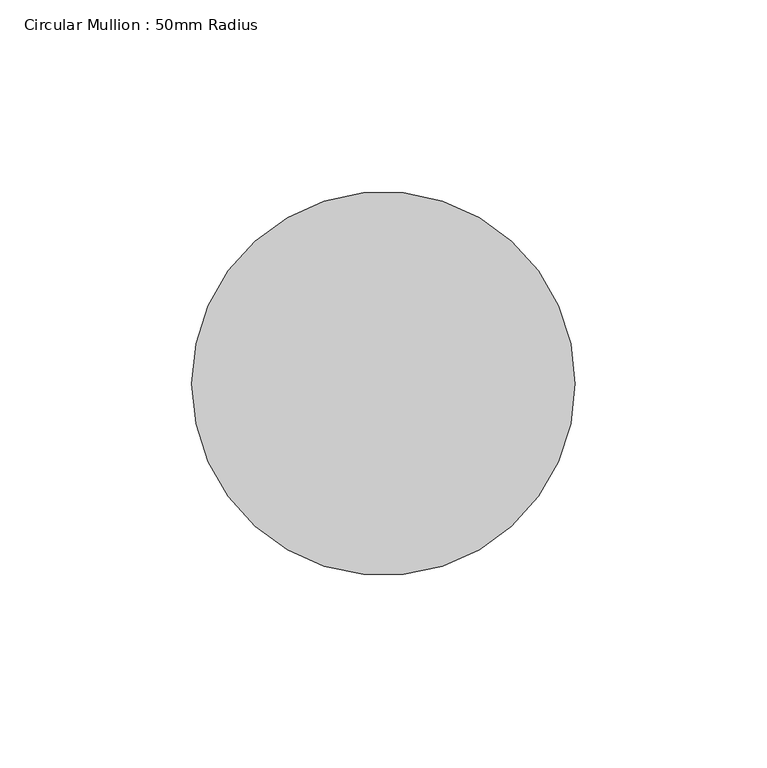
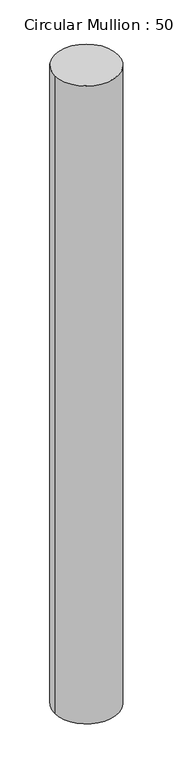
"""IFC4 building model written with IfcOpenShell, lengths in millimetres: member geometry, Circular Mullion : 50mm Radius."""

from ifc_helpers import new_model, si_unit, point, frame, origin, origin_2d, place, context, project, spatial, circle_curve, trimmed, segment, composite_curve, outline, extrude, source, transform, mapped, element, save


def circular_mullion_50mm_radius_614d2024(model_context):
    return source(origin(), model_context, "Body", "SweptSolid", [
        extrude(outline(composite_curve([segment(trimmed(circle_curve(origin_2d(), 50.0), [point((50.0, 0.0))], [point((-50.0, 0.0))], False, "CARTESIAN"), True, "CONTINUOUS"), segment(trimmed(circle_curve(origin_2d(), 50.0), [point((-50.0, 0.0))], [point((50.0, 0.0))], False, "CARTESIAN"), True, "CONTINUOUS")], self_intersect=False)), frame((0.0, 0.0, -1066.8394023), z_axis=(0.0, 0.0, 1.0), x_axis=(1.0, 0.0, 0.0)), (0.0, 0.0, 1.0), 1066.8394023),
    ])


if __name__ == "__main__":
    model = new_model("IFC4")
    model_context = context("Model", 3, world=origin())
    ifc_project = project(units=[si_unit("LENGTHUNIT", "METRE", prefix="MILLI")], contexts=[model_context])
    site = spatial("IfcSite", under=ifc_project)
    building = spatial("IfcBuilding", under=site)
    placement = place(None, origin())
    circular_mullion_50mm_radius_shape = circular_mullion_50mm_radius_614d2024(model_context)
    element("IfcMember", 1, ObjectType="Circular Mullion : 50mm Radius", at=placement, inside=building, context=model_context, shape_type="MappedRepresentation", body=[
        mapped(circular_mullion_50mm_radius_shape, transform((0.0, 0.0, 0.0), x_axis=(1.0, 0.0, 0.0), y_axis=(0.0, 1.0, 0.0), z_axis=(0.0, 0.0, 1.0))),
    ])
    save(model, "model.ifc")

# Revit data of these elements
# Type "Circular Mullion : 50mm Radius"
#   built-in parameter 1007350 = 0.164042 (stored number, unit not read)
# Element 1 (IfcMember, "Circular Mullion : 50mm Radius")
#   Materials on its faces: "Aluminium"
# Materials
#   "Aluminium": class "Metal", colour RGB 247 247 247, transparency 0, Description = "Aluminium 6061", Cost = 0
